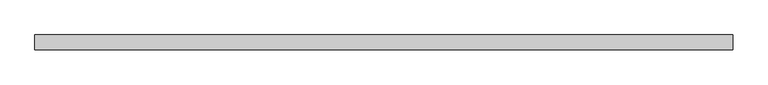
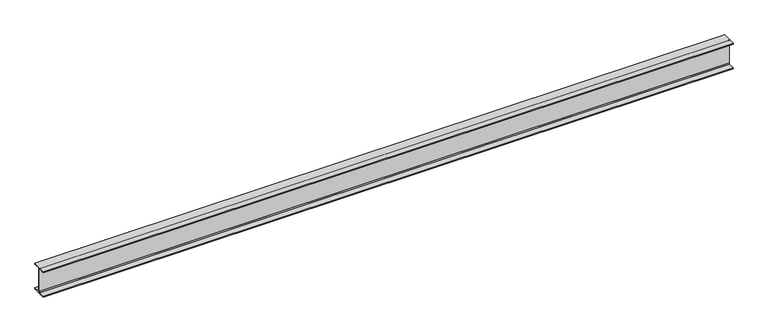
"""IFC4 building model written with IfcOpenShell, lengths in millimetres: beam geometry, Old_Steel Beam_H-KSD3502 : H_SB_ASB_H-400×200x8x13."""

from ifc_helpers import new_model, si_unit, point, frame, frame_2d, origin, place, context, project, spatial, polyline, circle_curve, trimmed, segment, composite_curve, outline, extrude, source, transform, mapped, element, save


def beam_8dad28fd(model_context):
    return source(origin(), model_context, "Body", "SweptSolid", [
        extrude(outline(composite_curve([segment(polyline([(82.5, -141.5), (82.5, -151.7), (-82.5, -151.7), (-82.5, -141.5), (-11.9, -141.5)]), True, "CONTINUOUS"), segment(trimmed(circle_curve(frame_2d((-11.9, -132.6)), 8.9), [point((-11.9, -141.5))], [point((-3.0, -132.6))], True, "CARTESIAN"), True, "CONTINUOUS"), segment(polyline([(-3.0, -132.6), (-3.0, 132.6)]), True, "CONTINUOUS"), segment(trimmed(circle_curve(frame_2d((-11.9, 132.6)), 8.9), [point((-3.0, 132.6))], [point((-11.9, 141.5))], True, "CARTESIAN"), True, "CONTINUOUS"), segment(polyline([(-11.9, 141.5), (-82.5, 141.5), (-82.5, 151.7), (82.5, 151.7), (82.5, 141.5), (11.9, 141.5)]), True, "CONTINUOUS"), segment(trimmed(circle_curve(frame_2d((11.9, 132.6)), 8.9), [point((11.9, 141.5))], [point((3.0, 132.6))], True, "CARTESIAN"), True, "CONTINUOUS"), segment(polyline([(3.0, 132.6), (3.0, -132.6)]), True, "CONTINUOUS"), segment(trimmed(circle_curve(frame_2d((11.9, -132.6)), 8.9), [point((3.0, -132.6))], [point((11.9, -141.5))], True, "CARTESIAN"), True, "CONTINUOUS"), segment(polyline([(11.9, -141.5), (82.5, -141.5)]), True, "CONTINUOUS")], self_intersect=False)), frame((-3904.8, 0.0, 0.0), z_axis=(1.0, 0.0, 0.0), x_axis=(0.0, 1.0, 0.0)), (0.0, 0.0, 1.0), 7809.6),
    ])


if __name__ == "__main__":
    model = new_model("IFC4")
    model_context = context("Model", 3, world=origin())
    ifc_project = project(units=[si_unit("LENGTHUNIT", "METRE", prefix="MILLI")], contexts=[model_context])
    site = spatial("IfcSite", under=ifc_project)
    building = spatial("IfcBuilding", under=site)
    placement = place(None, origin())
    beam_shape = beam_8dad28fd(model_context)
    element("IfcBeam", 1, ObjectType="Old_Steel Beam_H-KSD3502 : H_SB_ASB_H-400×200x8x13", at=placement, inside=building, context=model_context, shape_type="MappedRepresentation", body=[
        mapped(beam_shape, transform((0.0, 0.0, 0.0), x_axis=(1.0, 0.0, 0.0), y_axis=(0.0, 1.0, 0.0), z_axis=(0.0, 0.0, 1.0))),
    ])
    save(model, "model.ifc")

# Revit data of these elements
# Type "Old_Steel Beam_H-KSD3502 : H_SB_ASB_H-400×200x8x13"
#   Width = 20.0 cm
#   Web Thickness = 0.8 cm
#   Web Fillet = 1.6 cm
#   Warping Constant = 648999.0 cm⁶
#   Torsional Moment of Inertia = 35.8981 cm⁴
#   Torsional Modulus = 1.0 cm³
#   Section Area = 84.12 cm²
#   Plastic Modulus weak axis = 268.0 cm³
#   Plastic Modulus strong axis = 1330.0 cm³
#   Perimeter = 1.56 m²/m
#   Nominal Weight = 66.00 kgf/m
#   Moment of Inertia weak axis = 1740.00 cm⁴
#   Moment of Inertia strong axis = 23700.00 cm⁴
#   Height = 40.0 cm
#   Flange Thickness = 1.3 cm
#   Elastic Modulus weak axis = 174.0 cm³
#   Elastic Modulus strong axis = 1190.0 cm³
#   Centroid Vertical = 20.0 cm
#   Centroid Horizontal = 10.0 cm
#   Length [instance default] = 1.5240 m
#   Structural Material [instance default] = Steel, 45-345
#   Assembly Code = ""
# Element 1 (IfcBeam, "Old_Steel Beam_H-KSD3502 : H_SB_ASB_H-400×200x8x13")
#   Structural Material = none
# Materials
#   "Steel, 45-345": class "Metal", colour RGB 189 187 185, transparency 0, Description = "Steel 345 MPa", Cost = 0
